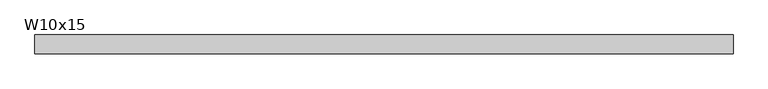
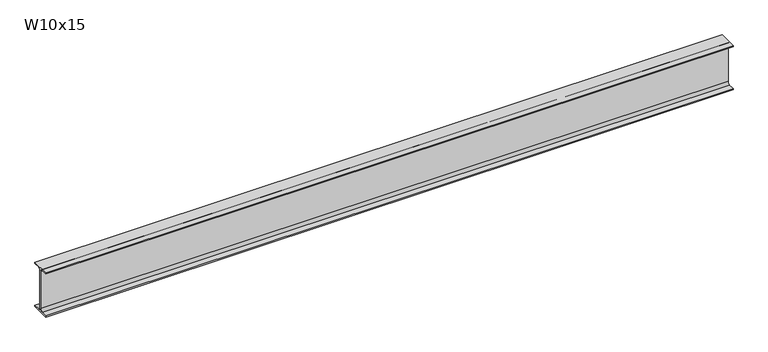
"""IFC4 building model written with IfcOpenShell, lengths in millimetres: beam geometry, RME W-Wide Flange : W10x15."""

from ifc_helpers import new_model, si_unit, point, frame, frame_2d, origin, place, context, project, spatial, polyline, circle_curve, trimmed, segment, composite_curve, outline, extrude, source, transform, mapped, element, save


def w10x15_21564ac7(model_context):
    return source(origin(), model_context, "Body", "SweptSolid", [
        extrude(outline(composite_curve([segment(polyline([(50.8, -120.142), (50.8, -127.0), (-50.8, -127.0), (-50.8, -120.142), (-16.7005, -120.142)]), True, "CONTINUOUS"), segment(trimmed(circle_curve(frame_2d((-16.7005, -106.3625)), 13.7795), [point((-16.7005, -120.142))], [point((-2.921, -106.3625))], True, "CARTESIAN"), True, "CONTINUOUS"), segment(polyline([(-2.921, -106.3625), (-2.921, 106.3625)]), True, "CONTINUOUS"), segment(trimmed(circle_curve(frame_2d((-16.7005, 106.3625)), 13.7795), [point((-2.921, 106.3625))], [point((-16.7005, 120.142))], True, "CARTESIAN"), True, "CONTINUOUS"), segment(polyline([(-16.7005, 120.142), (-50.8, 120.142), (-50.8, 127.0), (50.8, 127.0), (50.8, 120.142), (16.7005, 120.142)]), True, "CONTINUOUS"), segment(trimmed(circle_curve(frame_2d((16.7005, 106.3625)), 13.7795), [point((16.7005, 120.142))], [point((2.921, 106.3625))], True, "CARTESIAN"), True, "CONTINUOUS"), segment(polyline([(2.921, 106.3625), (2.921, -106.3625)]), True, "CONTINUOUS"), segment(trimmed(circle_curve(frame_2d((16.7005, -106.3625)), 13.7795), [point((2.921, -106.3625))], [point((16.7005, -120.142))], True, "CARTESIAN"), True, "CONTINUOUS"), segment(polyline([(16.7005, -120.142), (50.8, -120.142)]), True, "CONTINUOUS")], self_intersect=False)), frame((-1818.8305, 0.0, 0.0), z_axis=(1.0, 0.0, 0.0), x_axis=(0.0, 1.0, 0.0)), (0.0, 0.0, 1.0), 3732.9109994),
    ])


if __name__ == "__main__":
    model = new_model("IFC4")
    model_context = context("Model", 3, world=origin())
    ifc_project = project(units=[si_unit("LENGTHUNIT", "METRE", prefix="MILLI")], contexts=[model_context])
    site = spatial("IfcSite", under=ifc_project)
    building = spatial("IfcBuilding", under=site)
    placement = place(None, origin())
    w10x15_shape = w10x15_21564ac7(model_context)
    element("IfcBeam", 1, ObjectType="RME W-Wide Flange : W10x15", at=placement, inside=building, context=model_context, shape_type="MappedRepresentation", body=[
        mapped(w10x15_shape, transform((0.0, 0.0, 0.0), x_axis=(1.0, 0.0, 0.0), y_axis=(0.0, 1.0, 0.0), z_axis=(0.0, 0.0, 1.0))),
    ])
    save(model, "model.ifc")

# Revit data of these elements
# Type "RME W-Wide Flange : W10x15"
#   WELD P [instance default] = ""
#   WELD LE [instance default] = ""
#   WELD D [instance default] = ""
#   TOP SECTION SIZE [instance default] = ""
#   TOP SECTION LENGTH [instance default] = ""
#   REMARKS [instance default] = ""
#   REINF TYPE [instance default] = ""
#   Nominal Size = "W24"
#   End Bearing Capacity [instance default] = ""
#   BOT SECTION SIZE [instance default] = ""
#   BOT SECTION LENGTH [instance default] = ""
#   Assembly Code = "B10"
#   W = 15
#   Start Extension Calculation [instance default] = 10' - 0"
#   Start Extension [instance default] = -0' - 0 1/2"
#   End Extension Calculation [instance default] = 10' - 0"
#   End Extension [instance default] = -0' - 0 1/2"
#   Length [instance default] = 5' - 0"
#   bf = 0' - 4"
#   d = 0' - 10"
#   k = 0' - 0 13/16"
#   k2 = 0' - 0.5425"
#   tf = 0' - 0.27"
#   tw = 0' - 0.23"
#   A = 0.030625 SF
#   Structural Material [instance default] = Metal - Steel - ASTM A992
# Element 1 (IfcBeam, "RME W-Wide Flange : W10x15")
#   Length = 12' - 7.715"
#   Materials on its faces: "Metal - Steel - ASTM A992"
# Materials
#   "Metal - Steel - ASTM A992": class "Metal", colour RGB 255 128 0, transparency 0
